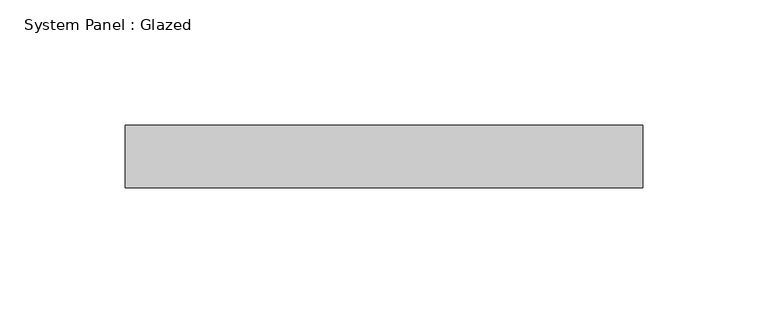
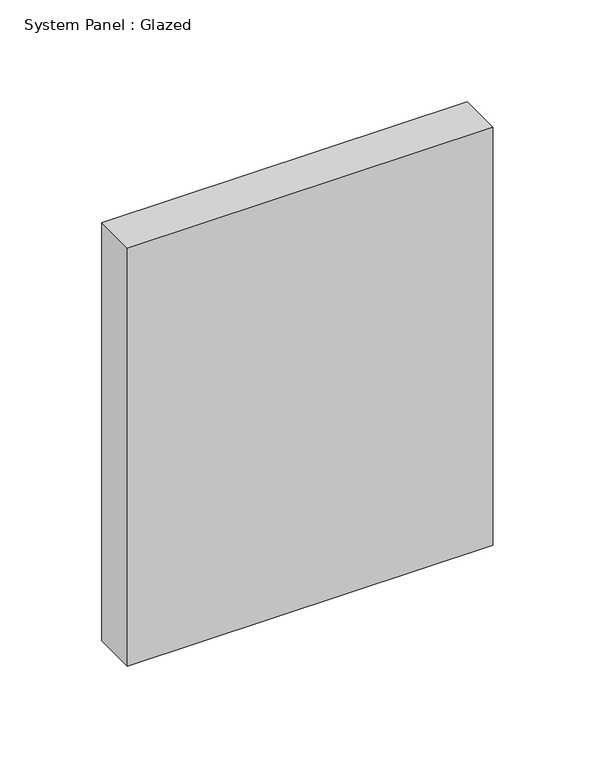
"""IFC4 building model written with IfcOpenShell, lengths in millimetres: plate geometry, System Panel : Glazed."""

from ifc_helpers import new_model, si_unit, origin, origin_with_axes, place, context, project, spatial, polyline, outline, extrude, source, transform, mapped, element, save


def system_panel_glazed_42eca631(model_context):
    return source(origin(), model_context, "Body", "SweptSolid", [
        extrude(outline(polyline([(103.4090909, 24.5), (-103.4090909, 24.5), (-103.4090909, 49.5), (103.4090909, 49.5), (103.4090909, 24.5)])), origin_with_axes(), (0.0, 0.0, 1.0), 250.0),
    ])


if __name__ == "__main__":
    model = new_model("IFC4")
    model_context = context("Model", 3, world=origin())
    ifc_project = project(units=[si_unit("LENGTHUNIT", "METRE", prefix="MILLI")], contexts=[model_context])
    site = spatial("IfcSite", under=ifc_project)
    building = spatial("IfcBuilding", under=site)
    placement = place(None, origin())
    system_panel_glazed_shape = system_panel_glazed_42eca631(model_context)
    element("IfcPlate", 1, ObjectType="System Panel : Glazed", at=placement, inside=building, context=model_context, shape_type="MappedRepresentation", body=[
        mapped(system_panel_glazed_shape, transform((0.0, 0.0, 0.0), x_axis=(1.0, 0.0, 0.0), y_axis=(0.0, 1.0, 0.0), z_axis=(0.0, 0.0, 1.0))),
    ])
    save(model, "model.ifc")

# Revit data of these elements
# Element 1 (IfcPlate, "System Panel : Glazed")
#   Materials on its faces: "Glass"
# Materials
#   "Glass": class "Glass", colour RGB 218 227 224, transparency 0.85, Description = "Soda Lime Glass", Cost = 0
